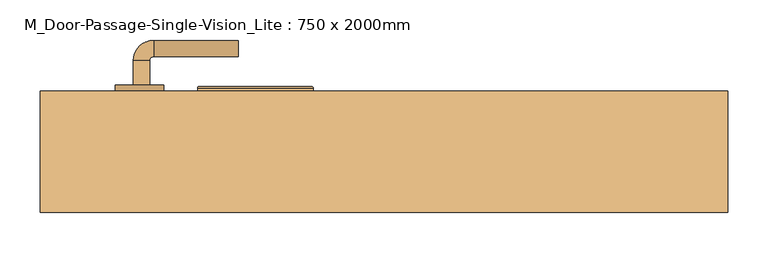
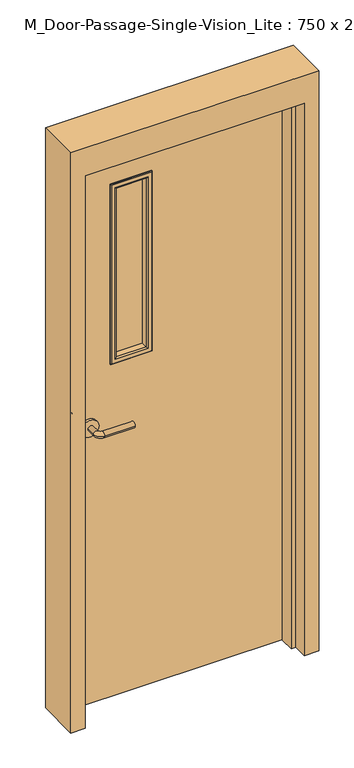
"""IFC4 building model written with IfcOpenShell, lengths in millimetres: door geometry, M_Door-Passage-Single-Vision_Lite : 750 x 2000mm."""

import ifcopenshell
import ifcopenshell.guid

model = None  # the IFC model being written
_history = None  # IfcOwnerHistory: only IFC2X3 demands one
_inside = {}  # id of a spatial element -> (the spatial element, [elements in it])
_under = {}  # id of a project, library or spatial element -> (it, [spatial elements below it])
_declared = {}  # id of a project -> (the project, [libraries it declares])
_typed = {}  # id of a type object -> (the type object, [elements of that type])
_made_of = {}  # id of a material, layer set ... -> (it, [elements and type objects made of it])


def new_model(schema):
    """Start an empty IFC model of exactly this schema.

    Asked for "IFC4X3", IfcOpenShell would pick the latest addendum, in which some entities
    have other attributes; the version numbers below select the first issue.
    IFC2X3 requires an IfcOwnerHistory on every rooted entity: one is made here for all.
    """
    global model, _history
    if schema == "IFC4X3":
        model = ifcopenshell.file(schema_version=(4, 3, 0, 0))
    else:
        model = ifcopenshell.file(schema=schema)
    _inside.clear()
    _under.clear()
    _declared.clear()
    _typed.clear()
    _made_of.clear()
    _history = None
    if model.schema == "IFC2X3":
        org = make("IfcOrganization", Name="unknown")
        user = make(
            "IfcPersonAndOrganization",
            ThePerson=make("IfcPerson", FamilyName="unknown"),
            TheOrganization=org,
        )
        app = make(
            "IfcApplication",
            ApplicationDeveloper=org,
            Version="unknown",
            ApplicationFullName="unknown",
            ApplicationIdentifier="unknown",
        )
        _history = make(
            "IfcOwnerHistory",
            OwningUser=user,
            OwningApplication=app,
            ChangeAction="ADDED",
            CreationDate=0,
        )
    return model


def make(cls, **values):
    """One entity of the class cls with the attributes given. An attribute that is None is left unset."""
    return model.create_entity(
        cls, **{name: value for name, value in values.items() if value is not None}
    )


def rooted(cls, **values):
    """An entity with a GlobalId (a new one), such as an element, a storey or a relation."""
    return make(cls, GlobalId=ifcopenshell.guid.new(), OwnerHistory=_history, **values)


def si_unit(unit_type, name, prefix=None):
    """IfcSIUnit, for example si_unit("LENGTHUNIT", "METRE", prefix="MILLI")."""
    return make("IfcSIUnit", UnitType=unit_type, Prefix=prefix, Name=name)


def assignment(units):
    """IfcUnitAssignment: the units of a project."""
    return None if units is None else make("IfcUnitAssignment", Units=units)


def point(xyz):
    """IfcCartesianPoint."""
    return None if xyz is None else make("IfcCartesianPoint", Coordinates=xyz)


def direction(xyz):
    """IfcDirection."""
    return None if xyz is None else make("IfcDirection", DirectionRatios=xyz)


def frame(location, z_axis=None, x_axis=None):
    """IfcAxis2Placement3D, a coordinate frame: its origin and axes. An axis left out is left unset."""
    return make(
        "IfcAxis2Placement3D",
        Location=point(location),
        Axis=direction(z_axis),
        RefDirection=direction(x_axis),
    )


def frame_2d(location, x_axis=None):
    """IfcAxis2Placement2D, a coordinate frame in the plane: its origin and x axis."""
    return make(
        "IfcAxis2Placement2D", Location=point(location), RefDirection=direction(x_axis)
    )


def origin():
    """The frame at (0, 0, 0) with its axes left unset."""
    return frame((0.0, 0.0, 0.0))


def place(relative_to, where):
    """IfcLocalPlacement: puts the frame where relative to a parent placement (None: the world)."""
    return make(
        "IfcLocalPlacement", PlacementRelTo=relative_to, RelativePlacement=where
    )


def context(
    kind, dimensions, precision=None, world=None, true_north=None, identifier=None
):
    """IfcGeometricRepresentationContext, for example the 3D "Model" context."""
    return make(
        "IfcGeometricRepresentationContext",
        ContextIdentifier=identifier,
        ContextType=kind,
        CoordinateSpaceDimension=dimensions,
        Precision=precision,
        WorldCoordinateSystem=world,
        TrueNorth=true_north,
    )


def project(units=None, contexts=None):
    """IfcProject with its units and contexts."""
    return rooted(
        "IfcProject",
        Name="project",
        RepresentationContexts=contexts,
        UnitsInContext=assignment(units),
    )


def spatial(cls, under=None, at=None, **own):
    """A site, building, storey or space (cls), placed at a placement, below another one or the project."""
    s = rooted(cls, ObjectPlacement=at, **own)
    if under is not None:
        _under.setdefault(under.id(), (under, []))[1].append(s)
    return s


def polyline(points):
    """IfcPolyline through the points."""
    return make("IfcPolyline", Points=[point(p) for p in points])


def circle_curve(where, radius):
    """IfcCircle in the frame where."""
    return make("IfcCircle", Position=where, Radius=radius)


def ellipse_curve(where, semi_axis1, semi_axis2):
    """IfcEllipse in the frame where."""
    return make(
        "IfcEllipse", Position=where, SemiAxis1=semi_axis1, SemiAxis2=semi_axis2
    )


def trimmed(basis, trim1, trim2, sense, master):
    """IfcTrimmedCurve: the piece of a basis curve between two trims."""
    return make(
        "IfcTrimmedCurve",
        BasisCurve=basis,
        Trim1=trim1,
        Trim2=trim2,
        SenseAgreement=sense,
        MasterRepresentation=master,
    )


def segment(curve, same_sense, transition):
    """IfcCompositeCurveSegment."""
    return make(
        "IfcCompositeCurveSegment",
        Transition=transition,
        SameSense=same_sense,
        ParentCurve=curve,
    )


def composite_curve(segments, self_intersect=None):
    """IfcCompositeCurve: segments joined end to end."""
    return make("IfcCompositeCurve", Segments=segments, SelfIntersect=self_intersect)


def outline(outer, holes=None, kind="AREA"):
    """IfcArbitraryClosedProfileDef: a profile drawn as a closed curve; with holes, ...WithVoids."""
    if holes is None:
        return make("IfcArbitraryClosedProfileDef", ProfileType=kind, OuterCurve=outer)
    return make(
        "IfcArbitraryProfileDefWithVoids",
        ProfileType=kind,
        OuterCurve=outer,
        InnerCurves=holes,
    )


def extrude(swept, where, along, depth):
    """IfcExtrudedAreaSolid: the profile swept, set in the frame where, extruded along a direction by depth."""
    return make(
        "IfcExtrudedAreaSolid",
        SweptArea=swept,
        Position=where,
        ExtrudedDirection=direction(along),
        Depth=depth,
    )


def faces_of(points, faces, orient=None, outer=None):
    """IfcFace entities. A face is a list of loops; a loop is a list of indices into points, from 0.

    orient and outer hold one flag for each loop. By default every Orientation is true, the
    first loop of a face is its IfcFaceOuterBound and the others are IfcFaceBound.
    """
    made = []
    for i, loops in enumerate(faces):
        bounds = []
        for j, loop in enumerate(loops):
            is_outer = j == 0 if outer is None else outer[i][j]
            bounds.append(
                make(
                    "IfcFaceOuterBound" if is_outer else "IfcFaceBound",
                    Bound=make("IfcPolyLoop", Polygon=[points[k] for k in loop]),
                    Orientation=True if orient is None else orient[i][j],
                )
            )
        made.append(make("IfcFace", Bounds=bounds))
    return made


def faceted_brep(points, faces, orient=None, outer=None, voids=None):
    """IfcFacetedBrep: a solid bounded by flat faces; with voids (closed shells), ...WithVoids."""
    shared = [point(p) for p in points]
    hull = make("IfcClosedShell", CfsFaces=faces_of(shared, faces, orient, outer))
    if voids is None:
        return make("IfcFacetedBrep", Outer=hull)
    return make(
        "IfcFacetedBrepWithVoids",
        Outer=hull,
        Voids=[
            make(cls, CfsFaces=faces_of(shared, fs, o, b)) for cls, fs, o, b in voids
        ],
    )


def shape(context_of_items, identifier, shape_type, items):
    """IfcShapeRepresentation: the items that make up one representation, for example the "Body"."""
    return make(
        "IfcShapeRepresentation",
        ContextOfItems=context_of_items,
        RepresentationIdentifier=identifier,
        RepresentationType=shape_type,
        Items=items,
    )


def source(mapping_origin, context_of_items, identifier, shape_type, items):
    """IfcRepresentationMap: a shape defined once, which mapped items show again and again."""
    return make(
        "IfcRepresentationMap",
        MappingOrigin=mapping_origin,
        MappedRepresentation=shape(context_of_items, identifier, shape_type, items),
    )


def transform(
    local_origin,
    x_axis=None,
    y_axis=None,
    z_axis=None,
    scale=None,
    scale2=None,
    scale3=None,
    uniform=True,
):
    """IfcCartesianTransformationOperator3D, or its non-uniform kind. x_axis, y_axis, z_axis: its Axis1, 2, 3."""
    if uniform:
        return make(
            "IfcCartesianTransformationOperator3D",
            Axis1=direction(x_axis),
            Axis2=direction(y_axis),
            LocalOrigin=point(local_origin),
            Scale=scale,
            Axis3=direction(z_axis),
        )
    return make(
        "IfcCartesianTransformationOperator3DnonUniform",
        Axis1=direction(x_axis),
        Axis2=direction(y_axis),
        LocalOrigin=point(local_origin),
        Scale=scale,
        Axis3=direction(z_axis),
        Scale2=scale2,
        Scale3=scale3,
    )


def mapped(mapping_source, mapping_target):
    """IfcMappedItem: shows the shape of a source again, moved by a transform."""
    return make(
        "IfcMappedItem", MappingSource=mapping_source, MappingTarget=mapping_target
    )


def made_of(thing, what):
    """Note that an element or type object is made of a material, layer set ...; save() writes the relation."""
    if what is not None:
        _made_of.setdefault(what.id(), (what, []))[1].append(thing)
    return thing


def element(
    cls,
    number,
    at=None,
    inside=None,
    cuts=None,
    type_object=None,
    material=None,
    context=None,
    identifier="Body",
    shape_type=None,
    held_by="IfcProductDefinitionShape",
    body=None,
    shapes=None,
    **own,
):
    """One element of the class cls, such as IfcWall. Its Tag is "e" and its number.

    at: its placement. inside: the storey or other place that contains it. cuts: it is an
    opening in that element (IfcRelVoidsElement). A single representation is given by context,
    identifier, shape_type and body (its items); several are given by shapes. held_by: the class
    of the entity that holds the representations. save() writes the other relations.
    """
    e = rooted(cls, Tag="e%d" % number, ObjectPlacement=at, **own)
    if body is not None:
        shapes = [shape(context, identifier, shape_type, body)]
    if shapes is not None:
        e.Representation = make(held_by, Representations=shapes)
    if inside is not None:
        _inside.setdefault(inside.id(), (inside, []))[1].append(e)
    if cuts is not None:
        rooted(
            "IfcRelVoidsElement", RelatingBuildingElement=cuts, RelatedOpeningElement=e
        )
    if type_object is not None:
        _typed.setdefault(type_object.id(), (type_object, []))[1].append(e)
    return made_of(e, material)


def aggregate(whole, parts):
    """IfcRelAggregates: a whole, such as a stair, and the parts it consists of."""
    return rooted("IfcRelAggregates", RelatingObject=whole, RelatedObjects=parts)


def save(model, path):
    """Write the relations noted so far, then the file.

    IfcRelAggregates (storeys below a building ...), IfcRelContainedInSpatialStructure (elements
    in a storey), IfcRelDefinesByType, IfcRelAssociatesMaterial and IfcRelDeclares: one each for
    every whole, place, type object, material and project.
    """
    for whole, parts in _under.values():
        aggregate(whole, parts)
    for where, things in _inside.values():
        rooted(
            "IfcRelContainedInSpatialStructure",
            RelatedElements=things,
            RelatingStructure=where,
        )
    for kind, things in _typed.values():
        rooted("IfcRelDefinesByType", RelatedObjects=things, RelatingType=kind)
    for what, things in _made_of.values():
        rooted("IfcRelAssociatesMaterial", RelatedObjects=things, RelatingMaterial=what)
    for by, libraries in _declared.values():
        rooted("IfcRelDeclares", RelatingContext=by, RelatedDefinitions=libraries)
    model.write(path)


def plane_surface(at):
    """IfcPlane: the flat surface through the origin of the frame at, square to its z axis."""
    return make("IfcPlane", Position=at)


def cylinder_surface(at, radius):
    """IfcCylindricalSurface: all points at the distance radius from the z axis of the frame at."""
    return make("IfcCylindricalSurface", Position=at, Radius=radius)


def revolved_surface(curve, axis_point, axis_direction):
    """IfcSurfaceOfRevolution: the curve turned about the line through axis_point along axis_direction."""
    return make(
        "IfcSurfaceOfRevolution",
        SweptCurve=make("IfcArbitraryOpenProfileDef", ProfileType="CURVE", Curve=curve),
        AxisPosition=make("IfcAxis1Placement", Location=point(axis_point), Axis=direction(axis_direction)),
    )


def advanced_brep(points, edges, surfaces, faces):
    """IfcAdvancedBrep: a solid bounded by faces that lie on surfaces and meet in shared edges.

    An edge is (start, end): straight between two places in points (the first is 0);
    or (start, end, curve); or (start, end, curve, False) where it runs against its curve.
    A face is (place in surfaces, loops), or (place, loops, False) where it looks against
    its surface's normal. A loop lists edges by number (the first is 1), with a minus sign
    where the edge is run from its end to its start. The first loop is the outer one.
    """
    corners = [point(p) for p in points]
    vertices = [make("IfcVertexPoint", VertexGeometry=c) for c in corners]
    made = []
    for start, end, *more in edges:
        made.append(
            make(
                "IfcEdgeCurve",
                EdgeStart=vertices[start],
                EdgeEnd=vertices[end],
                EdgeGeometry=more[0] if more else make("IfcPolyline", Points=[corners[start], corners[end]]),
                SameSense=more[1] if len(more) > 1 else True,
            )
        )
    hull = []
    for where, loops, *sense in faces:
        bounds = []
        for j, loop in enumerate(loops):
            ring = [make("IfcOrientedEdge", EdgeElement=made[abs(k) - 1], Orientation=k > 0) for k in loop]
            bounds.append(
                make(
                    "IfcFaceOuterBound" if j == 0 else "IfcFaceBound",
                    Bound=make("IfcEdgeLoop", EdgeList=ring),
                    Orientation=True,
                )
            )
        hull.append(make("IfcAdvancedFace", Bounds=bounds, FaceSurface=surfaces[where], SameSense=sense[0] if sense else True))
    return make("IfcAdvancedBrep", Outer=make("IfcClosedShell", CfsFaces=hull))


def m_door_passage_single_vision_lite_750_x_2000mm_4b244377(model_context):
    return source(origin(), model_context, "Body", "SolidModel", [
        advanced_brep(
        [(-309.990625, 3.35, 1000.0), (-289.990625, 3.35, 1000.0), (-289.990625, -26.65, 1000.0), (-309.990625, -26.65, 1000.0), (-284.990625, -31.65, 1000.0), (-284.990625, -51.65, 1000.0), (-179.990625, -51.65, 1000.0), (-179.990625, -31.65, 1000.0)],
        [
            (0, 1, circle_curve(frame((-299.990625, 3.35, 1000.0), z_axis=(0.0, 1.0, 0.0), x_axis=(1.0, 0.0, 0.0)), 10.0)),
            (1, 0, circle_curve(frame((-299.990625, 3.35, 1000.0), z_axis=(0.0, 1.0, 0.0), x_axis=(1.0, 0.0, 0.0)), 10.0)),
            (1, 2),
            (2, 3, circle_curve(frame((-299.990625, -26.65, 1000.0), z_axis=(0.0, 1.0, 0.0), x_axis=(1.0, 0.0, 0.0)), 10.0)),
            (3, 0),
            (3, 2, circle_curve(frame((-299.990625, -26.65, 1000.0), z_axis=(0.0, 1.0, 0.0), x_axis=(1.0, 0.0, 0.0)), 10.0)),
            (4, 5, circle_curve(frame((-284.990625, -41.65, 1000.0), z_axis=(-1.0, 0.0, 0.0), x_axis=(0.0, 1.0, 0.0)), 10.0)),
            (5, 3, circle_curve(frame((-284.990625, -26.65, 1000.0), z_axis=(0.0, 0.0, -1.0), x_axis=(-1.0, 0.0, 0.0)), 25.0)),
            (2, 4, circle_curve(frame((-284.990625, -26.65, 1000.0), z_axis=(0.0, 0.0, 1.0), x_axis=(-1.0, 0.0, 0.0)), 5.0)),
            (5, 4, circle_curve(frame((-284.990625, -41.65, 1000.0), z_axis=(-1.0, 0.0, 0.0), x_axis=(0.0, 1.0, 0.0)), 10.0)),
            (6, 7, circle_curve(frame((-179.990625, -41.65, 1000.0), z_axis=(1.0, 0.0, 0.0), x_axis=(0.0, 1.0, 0.0)), 10.0)),
            (7, 6, circle_curve(frame((-179.990625, -41.65, 1000.0), z_axis=(1.0, 0.0, 0.0), x_axis=(0.0, 1.0, 0.0)), 10.0)),
            (4, 7),
            (6, 5),
        ],
        [
            plane_surface(frame((-299.990625, 3.35, 1000.0), z_axis=(0.0, 1.0, 0.0), x_axis=(0.0, 0.0, 1.0))),
            cylinder_surface(frame((-299.990625, 3.35, 1000.0), z_axis=(0.0, 1.0, 0.0), x_axis=(1.0, 0.0, 0.0)), 10.0),
            revolved_surface(trimmed(ellipse_curve(frame((-299.990625, -26.65, 1000.0), z_axis=(0.0, -1.0, 0.0), x_axis=(1.0, 0.0, 0.0)), 10.0, 10.0), [point((-309.990625, -26.65, 1000.0))], [point((-289.990625, -26.65, 1000.0))], True, "CARTESIAN"), (-284.990625, -26.65, 1000.0), (0.0, 0.0, -1.0)),
            revolved_surface(trimmed(ellipse_curve(frame((-299.990625, -26.65, 1000.0), z_axis=(0.0, -1.0, 0.0), x_axis=(1.0, 0.0, 0.0)), 10.0, 10.0), [point((-289.990625, -26.65, 1000.0))], [point((-309.990625, -26.65, 1000.0))], True, "CARTESIAN"), (-284.990625, -26.65, 1000.0), (0.0, 0.0, -1.0)),
            plane_surface(frame((-179.990625, -41.65, 1000.0), z_axis=(1.0, 0.0, 0.0), x_axis=(0.0, 0.0, 1.0))),
            cylinder_surface(frame((-284.990625, -41.65, 1000.0), z_axis=(-1.0, 0.0, 0.0), x_axis=(0.0, 1.0, 0.0)), 10.0),
        ],
        [
            (0, [[1, 2]]),
            (1, [[3, 4, 5, -2]]),
            (1, [[-5, 6, -3, -1]]),
            (2, [[7, 8, -4, 9]]),
            (3, [[10, -9, -6, -8]]),
            (4, [[11, 12]]),
            (5, [[13, -11, 14, -7]]),
            (5, [[-14, -12, -13, -10]]),
        ],
    ),
        extrude(outline(composite_curve([segment(trimmed(circle_curve(frame_2d((1000.0, -302.490625)), 30.0), [point((1000.0, -332.490625))], [point((1000.0, -272.490625))], False, "CARTESIAN"), True, "CONTINUOUS"), segment(trimmed(circle_curve(frame_2d((1000.0, -302.490625)), 30.0), [point((1000.0, -272.490625))], [point((1000.0, -332.490625))], False, "CARTESIAN"), True, "CONTINUOUS")], self_intersect=False)), frame((0.0, 3.35, 0.0), z_axis=(0.0, 1.0, 0.0), x_axis=(0.0, 0.0, 1.0)), (0.0, 0.0, 1.0), 8.0),
        advanced_brep(
        [(-309.990625, 64.35, 1000.0), (-289.990625, 64.35, 1000.0), (-309.990625, 94.35, 1000.0), (-289.990625, 94.35, 1000.0), (-284.990625, 99.35, 1000.0), (-284.990625, 119.35, 1000.0), (-179.990625, 119.35, 1000.0), (-179.990625, 99.35, 1000.0)],
        [
            (0, 1, circle_curve(frame((-299.990625, 64.35, 1000.0), z_axis=(0.0, -1.0, 0.0), x_axis=(1.0, 0.0, 0.0)), 10.0)),
            (1, 0, circle_curve(frame((-299.990625, 64.35, 1000.0), z_axis=(0.0, -1.0, 0.0), x_axis=(1.0, 0.0, 0.0)), 10.0)),
            (0, 2),
            (2, 3, circle_curve(frame((-299.990625, 94.35, 1000.0), z_axis=(0.0, -1.0, 0.0), x_axis=(1.0, 0.0, 0.0)), 10.0)),
            (3, 1),
            (3, 2, circle_curve(frame((-299.990625, 94.35, 1000.0), z_axis=(0.0, -1.0, 0.0), x_axis=(1.0, 0.0, 0.0)), 10.0)),
            (4, 3, circle_curve(frame((-284.990625, 94.35, 1000.0), z_axis=(0.0, 0.0, 1.0), x_axis=(-1.0, 0.0, 0.0)), 5.0)),
            (2, 5, circle_curve(frame((-284.990625, 94.35, 1000.0), z_axis=(0.0, 0.0, -1.0), x_axis=(-1.0, 0.0, 0.0)), 25.0)),
            (5, 4, circle_curve(frame((-284.990625, 109.35, 1000.0), z_axis=(-1.0, 0.0, 0.0), x_axis=(0.0, -1.0, 0.0)), 10.0)),
            (4, 5, circle_curve(frame((-284.990625, 109.35, 1000.0), z_axis=(-1.0, 0.0, 0.0), x_axis=(0.0, -1.0, 0.0)), 10.0)),
            (6, 7, circle_curve(frame((-179.990625, 109.35, 1000.0), z_axis=(1.0, 0.0, 0.0), x_axis=(0.0, -1.0, 0.0)), 10.0)),
            (7, 6, circle_curve(frame((-179.990625, 109.35, 1000.0), z_axis=(1.0, 0.0, 0.0), x_axis=(0.0, -1.0, 0.0)), 10.0)),
            (5, 6),
            (7, 4),
        ],
        [
            plane_surface(frame((-299.990625, 64.35, 1000.0), z_axis=(0.0, -1.0, 0.0), x_axis=(0.0, 0.0, 1.0))),
            cylinder_surface(frame((-299.990625, 64.35, 1000.0), z_axis=(0.0, -1.0, 0.0), x_axis=(1.0, 0.0, 0.0)), 10.0),
            revolved_surface(trimmed(ellipse_curve(frame((-299.990625, 94.35, 1000.0), z_axis=(0.0, -1.0, 0.0), x_axis=(1.0, 0.0, 0.0)), 10.0, 10.0), [point((-309.990625, 94.35, 1000.0))], [point((-289.990625, 94.35, 1000.0))], True, "CARTESIAN"), (-284.990625, 94.35, 1000.0), (0.0, 0.0, -1.0)),
            revolved_surface(trimmed(ellipse_curve(frame((-299.990625, 94.35, 1000.0), z_axis=(0.0, -1.0, 0.0), x_axis=(1.0, 0.0, 0.0)), 10.0, 10.0), [point((-289.990625, 94.35, 1000.0))], [point((-309.990625, 94.35, 1000.0))], True, "CARTESIAN"), (-284.990625, 94.35, 1000.0), (0.0, 0.0, -1.0)),
            plane_surface(frame((-179.990625, 109.35, 1000.0), z_axis=(1.0, 0.0, 0.0), x_axis=(0.0, 0.0, 1.0))),
            cylinder_surface(frame((-284.990625, 109.35, 1000.0), z_axis=(-1.0, 0.0, 0.0), x_axis=(0.0, -1.0, 0.0)), 10.0),
        ],
        [
            (0, [[1, 2]]),
            (1, [[-1, 3, 4, 5]]),
            (1, [[-2, -5, 6, -3]]),
            (2, [[7, -4, 8, 9]]),
            (3, [[-8, -6, -7, 10]]),
            (4, [[11, 12]]),
            (5, [[-9, 13, -12, 14]]),
            (5, [[-10, -14, -11, -13]]),
        ],
    ),
        extrude(outline(composite_curve([segment(trimmed(circle_curve(frame_2d((1000.0, -302.490625)), 30.0), [point((1000.0, -332.490625))], [point((1000.0, -272.490625))], False, "CARTESIAN"), True, "CONTINUOUS"), segment(trimmed(circle_curve(frame_2d((1000.0, -302.490625)), 30.0), [point((1000.0, -272.490625))], [point((1000.0, -332.490625))], False, "CARTESIAN"), True, "CONTINUOUS")], self_intersect=False)), frame((0.0, 56.35, 0.0), z_axis=(0.0, 1.0, 0.0), x_axis=(0.0, 0.0, 1.0)), (0.0, 0.0, 1.0), 8.0),
        extrude(outline(polyline([(2000.0, -375.0), (0.0, -375.0), (0.0, 375.0), (2000.0, 375.0), (2000.0, -375.0)]), holes=[polyline([(1847.6, -222.6), (1847.6, -95.6), (1212.6, -95.6), (1212.6, -222.6), (1847.6, -222.6)])]), frame((0.0, 11.35, 0.0), z_axis=(0.0, 1.0, 0.0), x_axis=(0.0, 0.0, 1.0)), (0.0, 0.0, 1.0), 45.0),
        faceted_brep([(375.0, 6.5875, 0.0), (375.0, 56.35, 0.0), (425.0, 56.35, 0.0), (425.0, -93.65, 0.0), (375.0, -93.65, 0.0), (375.0, -44.4375, 0.0), (359.125, -44.4375, 0.0), (359.125, 6.5875, 0.0), (375.0, 6.5875, 2000.0), (375.0, 56.35, 2000.0), (-375.0, 56.35, 2000.0), (-375.0, 56.35, 0.0), (-425.0, 56.35, 0.0), (-425.0, 56.35, 2100.0), (425.0, 56.35, 2100.0), (425.0, -93.65, 2100.0), (-425.0, -93.65, 2100.0), (-425.0, -93.65, 0.0), (-375.0, -93.65, 0.0), (-375.0, -93.65, 2000.0), (375.0, -93.65, 2000.0), (375.0, -44.4375, 2000.0), (-375.0, -44.4375, 2000.0), (-375.0, -44.4375, 0.0), (-359.125, -44.4375, 0.0), (-359.125, -44.4375, 1984.125), (359.125, -44.4375, 1984.125), (359.125, 6.5875, 1984.125), (-359.125, 6.5875, 1984.125), (-359.125, 6.5875, 0.0), (-375.0, 6.5875, 0.0), (-375.0, 6.5875, 2000.0)], [[[0, 1, 2, 3, 4, 5, 6, 7]], [[1, 0, 8, 9]], [[2, 1, 9, 10, 11, 12, 13, 14]], [[3, 2, 14, 15]], [[4, 3, 15, 16, 17, 18, 19, 20]], [[5, 4, 20, 21]], [[6, 5, 21, 22, 23, 24, 25, 26]], [[7, 6, 26, 27]], [[0, 7, 27, 28, 29, 30, 31, 8]], [[9, 8, 31, 10]], [[20, 19, 22, 21]], [[26, 25, 28, 27]], [[12, 11, 30, 29, 24, 23, 18, 17]], [[11, 10, 31, 30]], [[13, 12, 17, 16]], [[19, 18, 23, 22]], [[25, 24, 29, 28]], [[15, 14, 13, 16]]]),
        extrude(outline(polyline([(-95.6, 31.35), (-222.6, 31.35), (-222.6, 36.35), (-95.6, 36.35), (-95.6, 31.35)])), frame((0.0, 0.0, 1212.6), z_axis=(0.0, 0.0, 1.0), x_axis=(1.0, 0.0, 0.0)), (0.0, 0.0, 1.0), 635.0),
        advanced_brep(
        [(-222.6, 36.35, 1847.6), (-222.6, 56.35, 1847.6), (-222.6, 56.35, 1212.6), (-222.6, 36.35, 1212.6), (-210.6, 57.35, 1835.6), (-210.6, 36.35, 1835.6), (-210.6, 36.35, 1224.6), (-210.6, 57.35, 1224.6), (-215.6, 62.35, 1840.6), (-215.6, 62.35, 1219.6), (-230.6, 60.35, 1855.6), (-228.6, 62.35, 1853.6), (-228.6, 62.35, 1206.6), (-230.6, 60.35, 1204.6), (-230.6, 56.35, 1855.6), (-230.6, 56.35, 1204.6), (-95.6, 56.35, 1212.6), (-95.6, 36.35, 1212.6), (-107.6, 36.35, 1224.6), (-107.6, 57.35, 1224.6), (-102.6, 62.35, 1219.6), (-89.6, 62.35, 1206.6), (-87.6, 60.35, 1204.6), (-87.6, 56.35, 1204.6), (-95.6, 56.35, 1847.6), (-95.6, 36.35, 1847.6), (-107.6, 36.35, 1835.6), (-107.6, 57.35, 1835.6), (-102.6, 62.35, 1840.6), (-89.6, 62.35, 1853.6), (-87.6, 60.35, 1855.6), (-87.6, 56.35, 1855.6)],
        [
            (0, 1),
            (1, 2),
            (2, 3),
            (3, 0),
            (4, 5),
            (5, 6),
            (6, 7),
            (7, 4),
            (8, 4, ellipse_curve(frame((-215.6, 57.35, 1840.6), z_axis=(-0.7071067811865475, 0.0, -0.7071067811865475), x_axis=(-0.7071067811865474, 0.0, 0.7071067811865476)), 7.0710678, 5.0)),
            (7, 9, ellipse_curve(frame((-215.6, 57.35, 1219.6), z_axis=(-0.7071067811865475, 0.0, 0.7071067811865475), x_axis=(0.7071067811865474, 0.0, 0.7071067811865476)), 7.0710678, 5.0)),
            (9, 8),
            (10, 11, ellipse_curve(frame((-228.6, 60.35, 1853.6), z_axis=(-0.7071067811865475, 0.0, -0.7071067811865475), x_axis=(-0.7071067811865474, 0.0, 0.7071067811865476)), 2.8284271, 2.0)),
            (11, 12),
            (12, 13, ellipse_curve(frame((-228.6, 60.35, 1206.6), z_axis=(-0.7071067811865475, 0.0, 0.7071067811865475), x_axis=(0.7071067811865474, 0.0, 0.7071067811865476)), 2.8284271, 2.0)),
            (13, 10),
            (14, 10),
            (13, 15),
            (15, 14),
            (2, 16),
            (16, 17),
            (17, 3),
            (6, 18),
            (18, 19),
            (19, 7),
            (19, 20, ellipse_curve(frame((-102.6, 57.35, 1219.6), z_axis=(-0.7071067811865475, 0.0, -0.7071067811865475), x_axis=(-0.7071067811865476, 0.0, 0.7071067811865474)), 7.0710678, 5.0)),
            (20, 9),
            (12, 21),
            (21, 22, ellipse_curve(frame((-89.6, 60.35, 1206.6), z_axis=(-0.7071067811865475, 0.0, -0.7071067811865475), x_axis=(-0.7071067811865476, 0.0, 0.7071067811865474)), 2.8284271, 2.0)),
            (22, 13),
            (22, 23),
            (23, 15),
            (16, 24),
            (24, 25),
            (25, 17),
            (18, 26),
            (26, 27),
            (27, 19),
            (27, 28, ellipse_curve(frame((-102.6, 57.35, 1840.6), z_axis=(0.7071067811865475, 0.0, -0.7071067811865475), x_axis=(-0.7071067811865474, 0.0, -0.7071067811865476)), 7.0710678, 5.0)),
            (28, 20),
            (21, 29),
            (29, 30, ellipse_curve(frame((-89.6, 60.35, 1853.6), z_axis=(0.7071067811865475, 0.0, -0.7071067811865475), x_axis=(-0.7071067811865474, 0.0, -0.7071067811865476)), 2.8284271, 2.0)),
            (30, 22),
            (30, 31),
            (31, 23),
            (31, 14),
            (1, 24),
            (0, 25),
            (5, 26),
            (4, 27),
            (8, 28),
            (11, 29),
            (10, 30),
        ],
        [
            plane_surface(frame((-222.6, 56.35, 1847.6), z_axis=(-1.0, 0.0, 0.0), x_axis=(0.0, 0.0, -1.0))),
            plane_surface(frame((-210.6, 36.35, 1835.6), z_axis=(1.0, 0.0, 0.0), x_axis=(0.0, 0.0, -1.0))),
            cylinder_surface(frame((-215.6, 57.35, 1847.6), z_axis=(0.0, 0.0, 1.0), x_axis=(-1.0, 0.0, 0.0)), 5.0),
            cylinder_surface(frame((-228.6, 60.35, 1847.6), z_axis=(0.0, 0.0, 1.0), x_axis=(-1.0, 0.0, 0.0)), 2.0),
            plane_surface(frame((-230.6, 60.35, 1855.6), z_axis=(-1.0, 0.0, 0.0), x_axis=(0.0, 0.0, -1.0))),
            plane_surface(frame((-222.6, 56.35, 1212.6), z_axis=(0.0, 0.0, -1.0), x_axis=(1.0, 0.0, 0.0))),
            plane_surface(frame((-210.6, 36.35, 1224.6), z_axis=(0.0, 0.0, 1.0), x_axis=(1.0, 0.0, 0.0))),
            cylinder_surface(frame((-222.6, 57.35, 1219.6), z_axis=(-1.0, 0.0, 0.0), x_axis=(0.0, 0.0, -1.0)), 5.0),
            cylinder_surface(frame((-222.6, 60.35, 1206.6), z_axis=(-1.0, 0.0, 0.0), x_axis=(0.0, 0.0, -1.0)), 2.0),
            plane_surface(frame((-230.6, 60.35, 1204.6), z_axis=(0.0, 0.0, -1.0), x_axis=(1.0, 0.0, 0.0))),
            plane_surface(frame((-95.6, 56.35, 1212.6), z_axis=(1.0, 0.0, 0.0), x_axis=(0.0, 0.0, 1.0))),
            plane_surface(frame((-107.6, 36.35, 1224.6), z_axis=(-1.0, 0.0, 0.0), x_axis=(0.0, 0.0, 1.0))),
            cylinder_surface(frame((-102.6, 57.35, 1212.6), z_axis=(0.0, 0.0, -1.0), x_axis=(1.0, 0.0, 0.0)), 5.0),
            cylinder_surface(frame((-89.6, 60.35, 1212.6), z_axis=(0.0, 0.0, -1.0), x_axis=(1.0, 0.0, 0.0)), 2.0),
            plane_surface(frame((-87.6, 60.35, 1204.6), z_axis=(1.0, 0.0, 0.0), x_axis=(0.0, 0.0, 1.0))),
            plane_surface(frame((-87.6, 56.35, 1855.6), z_axis=(0.0, -1.0, 0.0), x_axis=(-1.0, 0.0, 0.0))),
            plane_surface(frame((-95.6, 56.35, 1847.6), z_axis=(0.0, 0.0, 1.0), x_axis=(-1.0, 0.0, 0.0))),
            plane_surface(frame((-95.6, 36.35, 1847.6), z_axis=(0.0, -1.0, 0.0), x_axis=(-1.0, 0.0, 0.0))),
            plane_surface(frame((-107.6, 36.35, 1835.6), z_axis=(0.0, 0.0, -1.0), x_axis=(-1.0, 0.0, 0.0))),
            cylinder_surface(frame((-95.6, 57.35, 1840.6), z_axis=(1.0, 0.0, 0.0), x_axis=(0.0, 0.0, 1.0)), 5.0),
            plane_surface(frame((-102.6, 62.35, 1840.6), z_axis=(0.0, 1.0, 0.0), x_axis=(-1.0, 0.0, 0.0))),
            cylinder_surface(frame((-95.6, 60.35, 1853.6), z_axis=(1.0, 0.0, 0.0), x_axis=(0.0, 0.0, 1.0)), 2.0),
            plane_surface(frame((-87.6, 60.35, 1855.6), z_axis=(0.0, 0.0, 1.0), x_axis=(-1.0, 0.0, 0.0))),
        ],
        [
            (0, [[1, 2, 3, 4]]),
            (1, [[5, 6, 7, 8]]),
            (2, [[9, -8, 10, 11]]),
            (3, [[12, 13, 14, 15]]),
            (4, [[16, -15, 17, 18]]),
            (5, [[-3, 19, 20, 21]]),
            (6, [[-7, 22, 23, 24]]),
            (7, [[-10, -24, 25, 26]]),
            (8, [[-14, 27, 28, 29]]),
            (9, [[-17, -29, 30, 31]]),
            (10, [[-20, 32, 33, 34]]),
            (11, [[-23, 35, 36, 37]]),
            (12, [[-25, -37, 38, 39]]),
            (13, [[-28, 40, 41, 42]]),
            (14, [[-30, -42, 43, 44]]),
            (15, [[-31, -44, 45, -18], [46, -32, -19, -2]]),
            (16, [[-33, -46, -1, 47]]),
            (17, [[-21, -34, -47, -4], [48, -35, -22, -6]]),
            (18, [[-36, -48, -5, 49]]),
            (19, [[-38, -49, -9, 50]]),
            (20, [[51, -40, -27, -13], [-26, -39, -50, -11]]),
            (21, [[-41, -51, -12, 52]]),
            (22, [[-43, -52, -16, -45]]),
        ],
    ),
        advanced_brep(
        [(-222.6, 31.35, 1212.6), (-222.6, 11.35, 1212.6), (-222.6, 11.35, 1847.6), (-222.6, 31.35, 1847.6), (-210.6, 10.35, 1224.6), (-210.6, 31.35, 1224.6), (-210.6, 31.35, 1835.6), (-210.6, 10.35, 1835.6), (-215.6, 5.35, 1219.6), (-215.6, 5.35, 1840.6), (-230.6, 7.35, 1204.6), (-228.6, 5.35, 1206.6), (-228.6, 5.35, 1853.6), (-230.6, 7.35, 1855.6), (-230.6, 11.35, 1204.6), (-230.6, 11.35, 1855.6), (-95.6, 11.35, 1847.6), (-95.6, 31.35, 1847.6), (-107.6, 31.35, 1835.6), (-107.6, 10.35, 1835.6), (-102.6, 5.35, 1840.6), (-89.6, 5.35, 1853.6), (-87.6, 7.35, 1855.6), (-87.6, 11.35, 1855.6), (-95.6, 11.35, 1212.6), (-95.6, 31.35, 1212.6), (-107.6, 31.35, 1224.6), (-107.6, 10.35, 1224.6), (-102.6, 5.35, 1219.6), (-89.6, 5.35, 1206.6), (-87.6, 7.35, 1204.6), (-87.6, 11.35, 1204.6)],
        [
            (0, 1),
            (1, 2),
            (2, 3),
            (3, 0),
            (4, 5),
            (5, 6),
            (6, 7),
            (7, 4),
            (8, 4, ellipse_curve(frame((-215.6, 10.35, 1219.6), z_axis=(-0.7071067811865475, 0.0, 0.7071067811865475), x_axis=(-0.7071067811865474, 0.0, -0.7071067811865476)), 7.0710678, 5.0)),
            (7, 9, ellipse_curve(frame((-215.6, 10.35, 1840.6), z_axis=(-0.7071067811865475, 0.0, -0.7071067811865475), x_axis=(0.7071067811865474, 0.0, -0.7071067811865476)), 7.0710678, 5.0)),
            (9, 8),
            (10, 11, ellipse_curve(frame((-228.6, 7.35, 1206.6), z_axis=(-0.7071067811865475, 0.0, 0.7071067811865475), x_axis=(-0.7071067811865474, 0.0, -0.7071067811865476)), 2.8284271, 2.0)),
            (11, 12),
            (12, 13, ellipse_curve(frame((-228.6, 7.35, 1853.6), z_axis=(-0.7071067811865475, 0.0, -0.7071067811865475), x_axis=(0.7071067811865474, 0.0, -0.7071067811865476)), 2.8284271, 2.0)),
            (13, 10),
            (14, 10),
            (13, 15),
            (15, 14),
            (2, 16),
            (16, 17),
            (17, 3),
            (6, 18),
            (18, 19),
            (19, 7),
            (19, 20, ellipse_curve(frame((-102.6, 10.35, 1840.6), z_axis=(-0.7071067811865475, 0.0, 0.7071067811865475), x_axis=(-0.7071067811865476, 0.0, -0.7071067811865474)), 7.0710678, 5.0)),
            (20, 9),
            (12, 21),
            (21, 22, ellipse_curve(frame((-89.6, 7.35, 1853.6), z_axis=(-0.7071067811865475, 0.0, 0.7071067811865475), x_axis=(-0.7071067811865476, 0.0, -0.7071067811865474)), 2.8284271, 2.0)),
            (22, 13),
            (22, 23),
            (23, 15),
            (16, 24),
            (24, 25),
            (25, 17),
            (18, 26),
            (26, 27),
            (27, 19),
            (27, 28, ellipse_curve(frame((-102.6, 10.35, 1219.6), z_axis=(0.7071067811865475, 0.0, 0.7071067811865475), x_axis=(-0.7071067811865474, 0.0, 0.7071067811865476)), 7.0710678, 5.0)),
            (28, 20),
            (21, 29),
            (29, 30, ellipse_curve(frame((-89.6, 7.35, 1206.6), z_axis=(0.7071067811865475, 0.0, 0.7071067811865475), x_axis=(-0.7071067811865474, 0.0, 0.7071067811865476)), 2.8284271, 2.0)),
            (30, 22),
            (30, 31),
            (31, 23),
            (31, 14),
            (1, 24),
            (0, 25),
            (5, 26),
            (4, 27),
            (8, 28),
            (11, 29),
            (10, 30),
        ],
        [
            plane_surface(frame((-222.6, 11.35, 1212.6), z_axis=(-1.0, 0.0, 0.0), x_axis=(0.0, 0.0, 1.0))),
            plane_surface(frame((-210.6, 31.35, 1224.6), z_axis=(1.0, 0.0, 0.0), x_axis=(0.0, 0.0, 1.0))),
            cylinder_surface(frame((-215.6, 10.35, 1212.6), z_axis=(0.0, 0.0, -1.0), x_axis=(-1.0, 0.0, 0.0)), 5.0),
            cylinder_surface(frame((-228.6, 7.35, 1212.6), z_axis=(0.0, 0.0, -1.0), x_axis=(-1.0, 0.0, 0.0)), 2.0),
            plane_surface(frame((-230.6, 7.35, 1204.6), z_axis=(-1.0, 0.0, 0.0), x_axis=(0.0, 0.0, 1.0))),
            plane_surface(frame((-222.6, 11.35, 1847.6), z_axis=(0.0, 0.0, 1.0), x_axis=(1.0, 0.0, 0.0))),
            plane_surface(frame((-210.6, 31.35, 1835.6), z_axis=(0.0, 0.0, -1.0), x_axis=(1.0, 0.0, 0.0))),
            cylinder_surface(frame((-222.6, 10.35, 1840.6), z_axis=(-1.0, 0.0, 0.0), x_axis=(0.0, 0.0, 1.0)), 5.0),
            cylinder_surface(frame((-222.6, 7.35, 1853.6), z_axis=(-1.0, 0.0, 0.0), x_axis=(0.0, 0.0, 1.0)), 2.0),
            plane_surface(frame((-230.6, 7.35, 1855.6), z_axis=(0.0, 0.0, 1.0), x_axis=(1.0, 0.0, 0.0))),
            plane_surface(frame((-95.6, 11.35, 1847.6), z_axis=(1.0, 0.0, 0.0), x_axis=(0.0, 0.0, -1.0))),
            plane_surface(frame((-107.6, 31.35, 1835.6), z_axis=(-1.0, 0.0, 0.0), x_axis=(0.0, 0.0, -1.0))),
            cylinder_surface(frame((-102.6, 10.35, 1847.6), z_axis=(0.0, 0.0, 1.0), x_axis=(1.0, 0.0, 0.0)), 5.0),
            cylinder_surface(frame((-89.6, 7.35, 1847.6), z_axis=(0.0, 0.0, 1.0), x_axis=(1.0, 0.0, 0.0)), 2.0),
            plane_surface(frame((-87.6, 7.35, 1855.6), z_axis=(1.0, 0.0, 0.0), x_axis=(0.0, 0.0, -1.0))),
            plane_surface(frame((-87.6, 11.35, 1204.6), z_axis=(0.0, 1.0, 0.0), x_axis=(-1.0, 0.0, 0.0))),
            plane_surface(frame((-95.6, 11.35, 1212.6), z_axis=(0.0, 0.0, -1.0), x_axis=(-1.0, 0.0, 0.0))),
            plane_surface(frame((-95.6, 31.35, 1212.6), z_axis=(0.0, 1.0, 0.0), x_axis=(-1.0, 0.0, 0.0))),
            plane_surface(frame((-107.6, 31.35, 1224.6), z_axis=(0.0, 0.0, 1.0), x_axis=(-1.0, 0.0, 0.0))),
            cylinder_surface(frame((-95.6, 10.35, 1219.6), z_axis=(1.0, 0.0, 0.0), x_axis=(0.0, 0.0, -1.0)), 5.0),
            plane_surface(frame((-102.6, 5.35, 1219.6), z_axis=(0.0, -1.0, 0.0), x_axis=(-1.0, 0.0, 0.0))),
            cylinder_surface(frame((-95.6, 7.35, 1206.6), z_axis=(1.0, 0.0, 0.0), x_axis=(0.0, 0.0, -1.0)), 2.0),
            plane_surface(frame((-87.6, 7.35, 1204.6), z_axis=(0.0, 0.0, -1.0), x_axis=(-1.0, 0.0, 0.0))),
        ],
        [
            (0, [[1, 2, 3, 4]]),
            (1, [[5, 6, 7, 8]]),
            (2, [[9, -8, 10, 11]]),
            (3, [[12, 13, 14, 15]]),
            (4, [[16, -15, 17, 18]]),
            (5, [[-3, 19, 20, 21]]),
            (6, [[-7, 22, 23, 24]]),
            (7, [[-10, -24, 25, 26]]),
            (8, [[-14, 27, 28, 29]]),
            (9, [[-17, -29, 30, 31]]),
            (10, [[-20, 32, 33, 34]]),
            (11, [[-23, 35, 36, 37]]),
            (12, [[-25, -37, 38, 39]]),
            (13, [[-28, 40, 41, 42]]),
            (14, [[-30, -42, 43, 44]]),
            (15, [[-31, -44, 45, -18], [46, -32, -19, -2]]),
            (16, [[-33, -46, -1, 47]]),
            (17, [[-21, -34, -47, -4], [48, -35, -22, -6]]),
            (18, [[-36, -48, -5, 49]]),
            (19, [[-38, -49, -9, 50]]),
            (20, [[51, -40, -27, -13], [-26, -39, -50, -11]]),
            (21, [[-41, -51, -12, 52]]),
            (22, [[-43, -52, -16, -45]]),
        ],
    ),
    ])


if __name__ == "__main__":
    model = new_model("IFC4")
    model_context = context("Model", 3, world=origin())
    ifc_project = project(units=[si_unit("LENGTHUNIT", "METRE", prefix="MILLI")], contexts=[model_context])
    site = spatial("IfcSite", under=ifc_project)
    building = spatial("IfcBuilding", under=site)
    placement = place(None, origin())
    m_door_passage_single_vision_lite_750_x_2000mm_shape = m_door_passage_single_vision_lite_750_x_2000mm_4b244377(model_context)
    element("IfcDoor", 1, ObjectType="M_Door-Passage-Single-Vision_Lite : 750 x 2000mm", at=placement, inside=building, context=model_context, shape_type="MappedRepresentation", body=[
        mapped(m_door_passage_single_vision_lite_750_x_2000mm_shape, transform((0.0, 0.0, 0.0), x_axis=(1.0, 0.0, 0.0), y_axis=(0.0, 1.0, 0.0), z_axis=(0.0, 0.0, 1.0))),
    ])
    save(model, "model.ifc")

# Revit data of these elements
# Project information
#   Название организации = "Organization Name"
#   Описание организации = "Organization Description"
#   Наименование здания = "Building Name"
#   Дата утверждения проекта = "Issue Date"
#   Статус проекта = "Project Status"
#   Заказчик = "Client Name"
#   Адрес проекта = "Enter address here\nAddress Line 2"
#   Наименование проекта = "Project Name"
#   Номер проекта = "Project Number"
# Type "M_Door-Passage-Single-Vision_Lite : 750 x 2000mm"
#   Type Mark = "42"
#   Analytic Construction = "Wooden"
#   Thickness = 45 mm
#   Thermal Resistance (R) = 0.455703 (m²·K)/W
#   Swing Angle [instance default] = 90.00°
#   Strike Height = 1000 mm
#   Rough Width [instance default] = 850 mm
#   Rough Height [instance default] = 2100 mm
#   MFOpeningHeight [instance default] = 100 mm
#   MFOpeningWidth [instance default] = 100 mm
#   Inset Calculate [instance default] = 105 mm
#   Masonry Inset [instance default] = 25 mm
#   Height = 2000 mm
#   Width = 750 mm
#   Heat Transfer Coefficient (U) = 2.19465 W/(m²·K)
#   Masonry Frame Depth = 150 mm
#   Masonry Frame [instance default] = yes
#   Function = 1
#   Dry Wall Frame [instance default] = no
#   Panel Material = Wood - Birch
#   Glazing = Glass
#   Glass Stop Material = Metal - Paint Finish - Grey
#   Frame Material = Metal - Paint Finish - Grey
#   Door Handle Material = Aluminum
#   Visual Light Transmittance = 0
#   Solar Heat Gain Coefficient = 0
#   Wall Closure = (empty or 0)
# Element 1 (IfcDoor, "M_Door-Passage-Single-Vision_Lite : 750 x 2000mm")
#   Materials on its faces: "Metal - Paint Finish - Grey", "Aluminum", "Wood - Birch", "Glass"
# Materials
#   "Wood - Birch": class "Wood", colour RGB 173 132 96, transparency 0, Cost = 0
#   "Glass": class "Glass", colour RGB 245 245 243, transparency 1, Description = "Soda Lime Glass", Cost = 0
#   "Metal - Paint Finish - Grey": class "Paint", colour RGB 178 178 178, transparency 0, Cost = 0
#   "Aluminum": class "Metal", colour RGB 244 245 246, transparency 0, Description = "Aluminum 6061", Cost = 0
